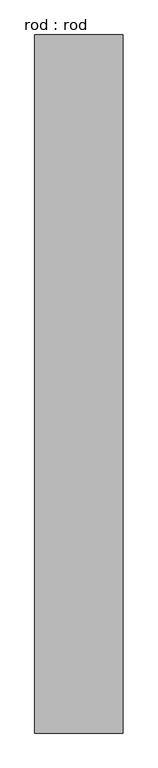
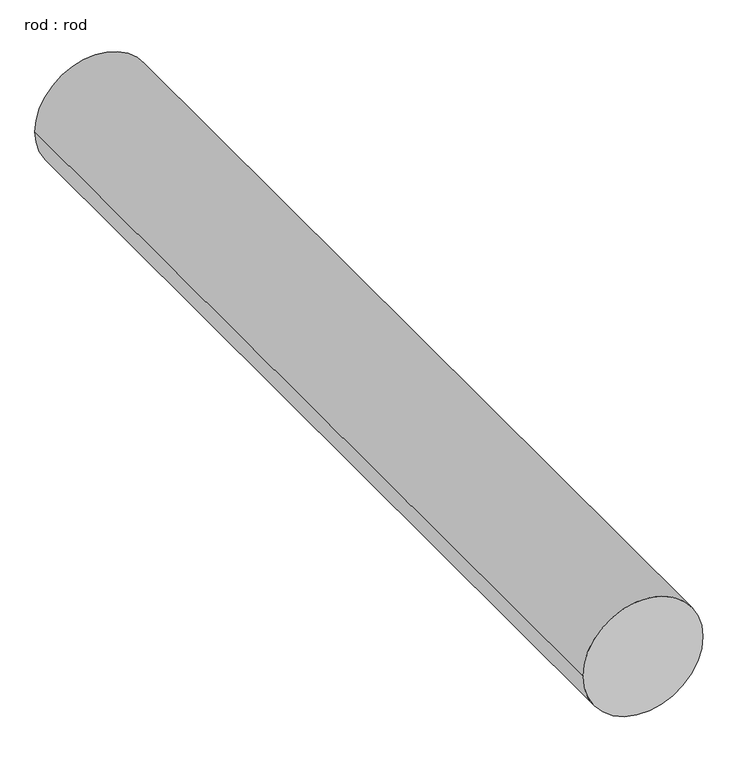
"""IFC4 building model written with IfcOpenShell, lengths in millimetres: proxy geometry, rod : rod."""

from ifc_helpers import new_model, si_unit, point, frame, frame_2d, origin, place, context, project, spatial, circle_curve, trimmed, segment, composite_curve, outline, extrude, source, transform, mapped, element, save


def rod_rod_9c36722f(model_context):
    return source(origin(), model_context, "Body", "SweptSolid", [
        extrude(outline(composite_curve([segment(trimmed(circle_curve(frame_2d((0.0108462, 0.0)), 200.0), [point((0.0108462, 200.0))], [point((0.0108462, -200.0))], False, "CARTESIAN"), True, "CONTINUOUS"), segment(trimmed(circle_curve(frame_2d((0.0108462, 0.0)), 200.0), [point((0.0108462, -200.0))], [point((0.0108462, 200.0))], False, "CARTESIAN"), True, "CONTINUOUS")], self_intersect=False)), frame((0.0, 2512.3714725, 0.0), z_axis=(0.0, 1.0, 0.0), x_axis=(0.0, 0.0, 1.0)), (0.0, 0.0, 1.0), 3160.7142857),
    ])


if __name__ == "__main__":
    model = new_model("IFC4")
    model_context = context("Model", 3, world=origin())
    ifc_project = project(units=[si_unit("LENGTHUNIT", "METRE", prefix="MILLI")], contexts=[model_context])
    site = spatial("IfcSite", under=ifc_project)
    building = spatial("IfcBuilding", under=site)
    placement = place(None, origin())
    rod_rod_shape = rod_rod_9c36722f(model_context)
    element("IfcBuildingElementProxy", 1, Name="rod : rod", ObjectType="rod : rod", at=placement, inside=building, context=model_context, shape_type="MappedRepresentation", body=[
        mapped(rod_rod_shape, transform((0.0, 0.0, 0.0), x_axis=(1.0, 0.0, 0.0), y_axis=(0.0, 1.0, 0.0), z_axis=(0.0, 0.0, 1.0))),
    ])
    save(model, "model.ifc")

# Revit data of these elements
# Type "rod : rod"
#   Default Elevation = 0
